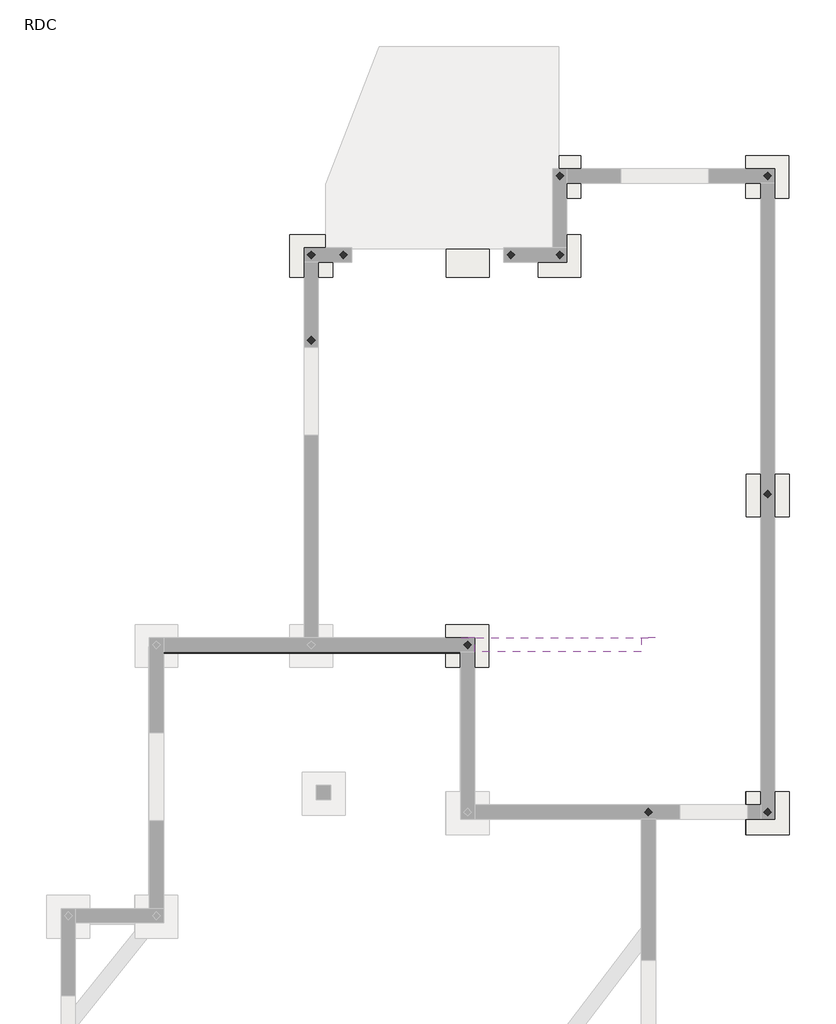
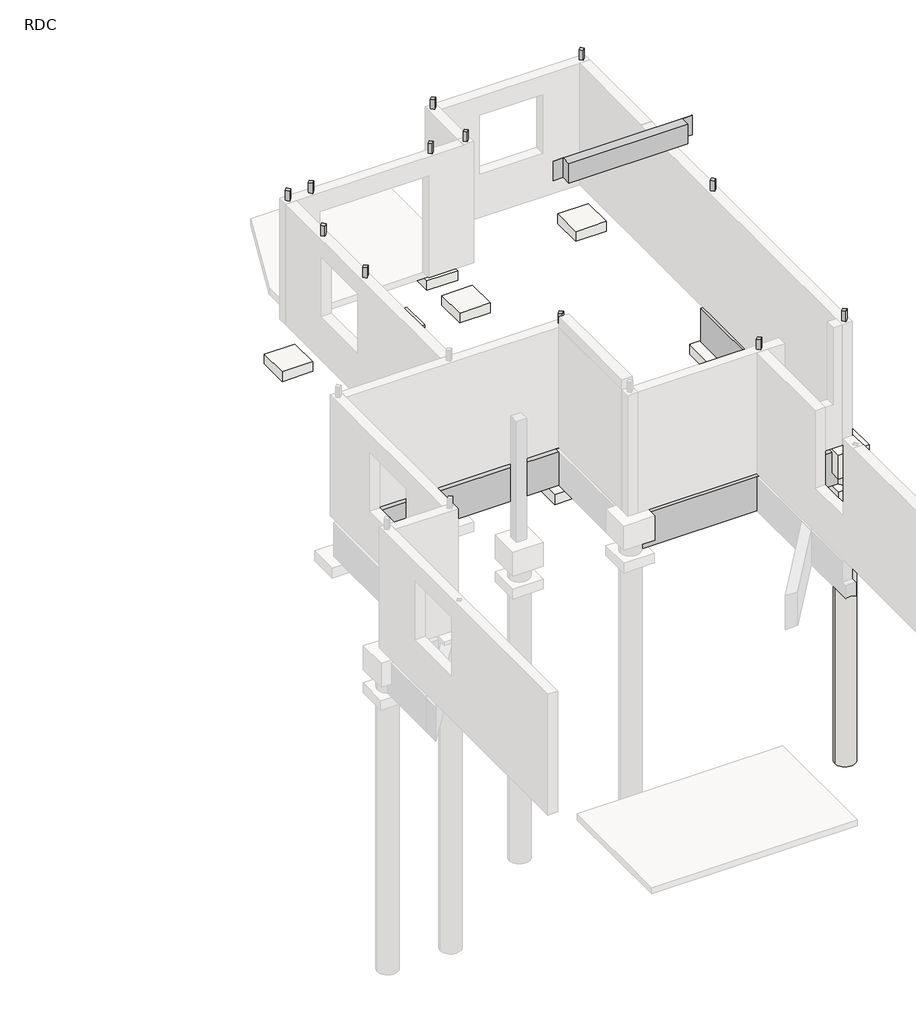
# One storey, part 5 of 5: 12 columns, 10 slabs, 4 beams.
"""IFC4 building model written with IfcOpenShell, lengths in millimetres."""

from ifc_helpers import new_model, si_unit, frame, origin, place, context, project, spatial, polyline, circle_curve, outline, extrude, faceted_brep, element, save
from ifc_brep_helpers import plane_surface, cylinder_surface, revolved_surface, advanced_brep

model = new_model("IFC4")

# Units and contexts
model_context = context("Model", 3, world=origin())
ifc_project = project(units=[si_unit("LENGTHUNIT", "METRE", prefix="MILLI")], contexts=[model_context])

# Site, building, storey
site = spatial("IfcSite", under=ifc_project)
building = spatial("IfcBuilding", under=site)
storey = spatial("IfcBuildingStorey", under=building, Name="RDC", Elevation=0.0)

# Beams
placement = place(None, origin())
element("IfcBeam", 1, ObjectType="Longrine BA : 20x70ht", at=placement, inside=storey, context=model_context, shape_type="AdvancedBrep", body=[
    advanced_brep(
    [(3744.5663998, 5403.8353673, -67.0), (3744.5663998, 5403.8353673, -767.0), (3740.0228667, 5403.8353673, -767.0), (3740.0228667, 5403.8353673, -67.0), (3744.5663998, 808.0224787, -67.0), (3744.5663998, 808.0224787, -500.0), (3744.5663998, 681.2275595, -500.0), (3744.5663998, 681.2275595, -767.0), (3544.5663998, 681.2275595, -767.0), (3544.5663998, 5213.5020686, -767.0), (3740.0228667, 5213.5020686, -767.0), (3544.5663998, 681.2275595, -500.0), (3544.5663998, 808.0224787, -500.0), (3544.5663998, 808.0224787, -67.0), (3544.5663998, 5213.5020686, -67.0), (3740.0228667, 5213.5020686, -67.0)],
    [
        (0, 1),
        (1, 2),
        (2, 3),
        (3, 0),
        (0, 4),
        (4, 5),
        (5, 6),
        (6, 7),
        (7, 1),
        (7, 8, circle_curve(frame((3644.5663998, 508.0224787, -767.0), z_axis=(0.0, 0.0, 1.0), x_axis=(1.0, 0.0, 0.0)), 200.0)),
        (8, 9),
        (9, 10),
        (10, 2),
        (8, 11),
        (11, 12),
        (12, 13),
        (13, 14),
        (14, 9),
        (3, 15),
        (15, 14),
        (13, 4),
        (6, 11, circle_curve(frame((3644.5663998, 508.0224787, -500.0), z_axis=(0.0, 0.0, 1.0), x_axis=(1.0, 0.0, 0.0)), 200.0)),
        (5, 12),
        (10, 15),
    ],
    [
        plane_surface(frame((3744.5663998, 5403.8353673, -67.0), z_axis=(0.0, 1.0, 0.0), x_axis=(0.0, 0.0, -1.0))),
        plane_surface(frame((3744.5663998, 5403.8353673, -417.0), z_axis=(1.0, 0.0, 0.0), x_axis=(0.0, 0.0, -1.0))),
        plane_surface(frame((3644.5663998, 5403.8353673, -767.0), z_axis=(0.0, 0.0, -1.0), x_axis=(-1.0, 0.0, 0.0))),
        plane_surface(frame((3544.5663998, 5403.8353673, -417.0), z_axis=(-1.0, 0.0, 0.0), x_axis=(0.0, 0.0, 1.0))),
        plane_surface(frame((3644.5663998, 5403.8353673, -67.0), z_axis=(0.0, 0.0, 1.0), x_axis=(1.0, 0.0, 0.0))),
        revolved_surface(polyline([(3844.5663998, 508.0224787, -500.0), (3844.5663998, 508.0224787, -767.0)]), (3644.5663998, 508.0224787, -6600.0), (0.0, 0.0, 1.0)),
        plane_surface(frame((3344.5663998, 808.0224787, -500.0), z_axis=(0.0, 0.0, 1.0), x_axis=(1.0, 0.0, 0.0))),
        plane_surface(frame((3944.5663998, 808.0224787, 0.0), z_axis=(0.0, -1.0, 0.0), x_axis=(0.0, 0.0, -1.0))),
        plane_surface(frame((3740.0228667, 9413.5020686, -770.0), z_axis=(-1.0, 0.0, 0.0), x_axis=(0.0, 1.0, 0.0))),
        plane_surface(frame((3540.0228667, 5213.5020686, -770.0), z_axis=(0.0, 1.0, 0.0), x_axis=(1.0, 0.0, 0.0))),
    ],
    [
        (0, [[1, 2, 3, 4]]),
        (1, [[-1, 5, 6, 7, 8, 9]]),
        (2, [[-9, 10, 11, 12, 13, -2]]),
        (3, [[14, 15, 16, 17, 18, -11]]),
        (4, [[-5, -4, 19, 20, -17, 21]]),
        (5, [[-10, -8, 22, -14]]),
        (6, [[23, -15, -22, -7]]),
        (7, [[-23, -6, -21, -16]]),
        (8, [[24, -19, -3, -13]]),
        (9, [[-24, -12, -18, -20]]),
    ],
),
])
element("IfcBeam", 2, ObjectType="Longrine BA : 20x70ht", at=placement, inside=storey, context=model_context, shape_type="AdvancedBrep", body=[
    advanced_brep(
    [(3463.1482907, 423.8353673, -767.0), (3463.1482907, 423.8353673, -500.0), (3344.5663998, 423.8353673, -500.0), (3344.5663998, 423.8353673, -67.0), (2074.5663639, 423.8353673, -67.0), (1874.5663639, 423.8353673, -67.0), (-255.4335965, 423.8353673, -67.0), (-255.4335965, 423.8353673, -500.0), (-374.0154875, 423.8353673, -500.0), (-374.0154875, 423.8353673, -767.0), (1874.5663639, 423.8353673, -767.0), (2074.5663639, 423.8353673, -767.0), (-355.4335965, 508.0224787, -767.0), (-392.3772418, 623.8353673, -767.0), (3481.510045, 623.8353673, -767.0), (3444.5663998, 508.0224787, -767.0), (3481.510045, 623.8353673, -500.0), (-392.3772418, 623.8353673, -500.0), (-255.4335965, 623.8353673, -500.0), (-255.4335965, 623.8353673, -67.0), (3344.5663998, 623.8353673, -67.0), (3344.5663998, 623.8353673, -500.0), (-355.4335965, 508.0224787, -500.0), (3444.5663998, 508.0224787, -500.0)],
    [
        (0, 1),
        (1, 2),
        (2, 3),
        (3, 4),
        (4, 5),
        (5, 6),
        (6, 7),
        (7, 8),
        (8, 9),
        (9, 10),
        (10, 11),
        (11, 0),
        (9, 12, circle_curve(frame((-555.4335965, 508.0224787, -767.0), z_axis=(0.0, 0.0, 1.0), x_axis=(1.0, 0.0, 0.0)), 200.0)),
        (12, 13, circle_curve(frame((-555.4335965, 508.0224787, -767.0), z_axis=(0.0, 0.0, 1.0), x_axis=(1.0, 0.0, 0.0)), 200.0)),
        (13, 14),
        (14, 15, circle_curve(frame((3644.5663998, 508.0224787, -767.0), z_axis=(0.0, 0.0, 1.0), x_axis=(1.0, 0.0, 0.0)), 200.0)),
        (15, 0, circle_curve(frame((3644.5663998, 508.0224787, -767.0), z_axis=(0.0, 0.0, 1.0), x_axis=(1.0, 0.0, 0.0)), 200.0)),
        (16, 14),
        (13, 17),
        (17, 18),
        (18, 19),
        (19, 20),
        (20, 21),
        (21, 16),
        (3, 20),
        (19, 6),
        (8, 22, circle_curve(frame((-555.4335965, 508.0224787, -500.0), z_axis=(0.0, 0.0, 1.0), x_axis=(1.0, 0.0, 0.0)), 200.0)),
        (22, 12),
        (22, 17, circle_curve(frame((-555.4335965, 508.0224787, -500.0), z_axis=(0.0, 0.0, 1.0), x_axis=(1.0, 0.0, 0.0)), 200.0)),
        (15, 23),
        (23, 1, circle_curve(frame((3644.5663998, 508.0224787, -500.0), z_axis=(0.0, 0.0, 1.0), x_axis=(1.0, 0.0, 0.0)), 200.0)),
        (16, 23, circle_curve(frame((3644.5663998, 508.0224787, -500.0), z_axis=(0.0, 0.0, 1.0), x_axis=(1.0, 0.0, 0.0)), 200.0)),
        (21, 2),
        (7, 18),
    ],
    [
        plane_surface(frame((3631.8663992, 423.8353673, -417.0), z_axis=(0.0, -1.0, 0.0), x_axis=(0.0, 0.0, -1.0))),
        plane_surface(frame((3631.8663992, 523.8353673, -767.0), z_axis=(0.0, 0.0, -1.0), x_axis=(0.0, 1.0, 0.0))),
        plane_surface(frame((3631.8663992, 623.8353673, -417.0), z_axis=(0.0, 1.0, 0.0), x_axis=(0.0, 0.0, 1.0))),
        plane_surface(frame((3631.8663992, 523.8353673, -67.0), z_axis=(0.0, 0.0, 1.0), x_axis=(0.0, -1.0, 0.0))),
        revolved_surface(polyline([(-355.4335965, 508.0224787, -500.0), (-355.4335965, 508.0224787, -767.0)]), (-555.4335965, 508.0224787, -6600.0), (0.0, 0.0, 1.0)),
        revolved_surface(polyline([(3844.5663998, 508.0224787, -500.0), (3844.5663998, 508.0224787, -767.0)]), (3644.5663998, 508.0224787, -6600.0), (0.0, 0.0, 1.0)),
        plane_surface(frame((3344.5663998, 808.0224787, -500.0), z_axis=(0.0, 0.0, 1.0), x_axis=(1.0, 0.0, 0.0))),
        plane_surface(frame((3344.5663998, 808.0224787, 0.0), z_axis=(1.0, 0.0, 0.0), x_axis=(0.0, 0.0, -1.0))),
        plane_surface(frame((-855.4335965, 808.0224787, -500.0), z_axis=(0.0, 0.0, 1.0), x_axis=(1.0, 0.0, 0.0))),
        plane_surface(frame((-255.4335965, 208.0224787, 0.0), z_axis=(-1.0, 0.0, 0.0), x_axis=(0.0, 0.0, -1.0))),
    ],
    [
        (0, [[1, 2, 3, 4, 5, 6, 7, 8, 9, 10, 11, 12]]),
        (1, [[13, 14, 15, 16, 17, -12, -11, -10]]),
        (2, [[18, -15, 19, 20, 21, 22, 23, 24]]),
        (3, [[25, -22, 26, -6, -5, -4]]),
        (4, [[-13, -9, 27, 28]]),
        (4, [[-14, -28, 29, -19]]),
        (5, [[-1, -17, 30, 31]]),
        (5, [[-18, 32, -30, -16]]),
        (6, [[33, -2, -31, -32, -24]]),
        (7, [[-33, -23, -25, -3]]),
        (8, [[34, -20, -29, -27, -8]]),
        (9, [[-34, -7, -26, -21]]),
    ],
),
])
element("IfcBeam", 3, ObjectType="Longrine BA : 20x70ht", at=placement, inside=storey, context=model_context, shape_type="Brep", body=[
    faceted_brep([(-4904.4649416, 2948.0224782, -67.0), (-4904.4649416, 2948.0224782, -767.0), (-4904.4649416, 2835.3224776, -767.0), (-4904.4649416, 2835.3224776, -67.0), (-572.6771131, 2948.0224782, -67.0), (-572.6771131, 2835.3224776, -67.0), (-572.6771131, 2748.0224782, -67.0), (-572.6771131, 2748.0224782, -767.0), (-572.6771131, 2835.3224776, -767.0), (-572.6771131, 2948.0224782, -767.0), (-2849.9542111, 2948.0224782, -67.0), (-2849.9542111, 2948.0224782, -767.0), (-659.9771125, 2748.0224782, -767.0), (-4817.1649422, 2748.0224782, -767.0), (-4817.1649422, 2835.3224776, -767.0), (-2849.9542111, 2947.3616236, -767.0), (-2649.9542111, 2947.3616236, -767.0), (-2649.9542111, 2948.0224782, -767.0), (-659.9771125, 2748.0224782, -67.0), (-4817.1649422, 2748.0224782, -67.0), (-2649.9542111, 2948.0224782, -67.0), (-2649.9542111, 2947.3616236, -67.0), (-2849.9542111, 2947.3616236, -67.0), (-4817.1649422, 2835.3224776, -67.0)], [[[0, 1, 2, 3]], [[4, 5, 6, 7, 8, 9]], [[1, 0, 10, 11]], [[9, 8, 7, 12, 13, 14, 2, 1, 11, 15, 16, 17]], [[7, 6, 18, 19, 13, 12]], [[6, 5, 4, 20, 21, 22, 10, 0, 3, 23, 19, 18]], [[23, 14, 13, 19]], [[14, 23, 3, 2]], [[22, 15, 11, 10]], [[15, 22, 21, 16]], [[4, 9, 17, 20]], [[16, 21, 20, 17]]]),
])
element("IfcBeam", 4, ObjectType="Poutres BA : 20x40h", at=placement, inside=storey, context=model_context, shape_type="SweptSolid", body=[
    extrude(outline(polyline([(-645.8307775, 2964.0588408), (2074.1692225, 2964.0588408), (2074.1692225, 2963.8353669), (1874.5663639, 2963.8353669), (1874.5663639, 2764.0588408), (-455.4335965, 2764.0588408), (-455.4335965, 2963.8353669), (-645.8307775, 2963.8353669), (-645.8307775, 2964.0588408)])), frame((0.0, 0.0, 5410.0), z_axis=(0.0, 0.0, 1.0), x_axis=(1.0, 0.0, 0.0)), (0.0, 0.0, 1.0), 400.0),
])

# Columns
element("IfcColumn", 5, ObjectType="CV : CV", at=placement, inside=storey, context=model_context, shape_type="Brep", body=[
    faceted_brep([(-555.4335965, 2916.8683755, 2710.0), (-608.4666051, 2863.8353669, 2710.0), (-555.4335965, 2810.8023583, 2710.0), (-502.4005879, 2863.8353669, 2710.0), (-555.4335965, 2916.8683755, 0.0), (-502.4005879, 2863.8353669, 0.0), (-555.4335965, 2810.8023583, 0.0), (-608.4666051, 2863.8353669, 0.0), (-555.4335965, 2916.8683755, 2500.0), (-608.4666051, 2863.8353669, 2500.0), (-555.4335965, 2810.8023583, 2500.0), (-502.4005879, 2863.8353669, 2500.0)], [[[0, 1, 2, 3]], [[4, 5, 6, 7]], [[1, 0, 8, 4, 7, 9]], [[2, 1, 9, 7, 6, 10]], [[3, 2, 10, 6, 5, 11]], [[0, 3, 11, 5, 4, 8]]]),
    faceted_brep([(-502.4005879, 2863.8353669, 2710.0), (-555.4335965, 2916.8683755, 2710.0), (-608.4666051, 2863.8353669, 2710.0), (-555.4335965, 2810.8023583, 2710.0), (-502.4005879, 2863.8353669, 0.0), (-555.4335965, 2810.8023583, 0.0), (-608.4666051, 2863.8353669, 0.0), (-555.4335965, 2916.8683755, 0.0), (-502.4005879, 2863.8353669, 2500.0), (-555.4335965, 2916.8683755, 2500.0), (-608.4666051, 2863.8353669, 2500.0), (-555.4335965, 2810.8023583, 2500.0)], [[[0, 1, 2, 3]], [[4, 5, 6, 7]], [[1, 0, 8, 4, 7, 9]], [[2, 1, 9, 7, 6, 10]], [[3, 2, 10, 6, 5, 11]], [[0, 3, 11, 5, 4, 8]]]),
])
element("IfcColumn", 6, ObjectType="CV : CV", at=placement, inside=storey, context=model_context, shape_type="Brep", body=[
    faceted_brep([(-2745.4336004, 5751.8684051, 2710.0), (-2798.466609, 5698.8353965, 2710.0), (-2745.4336004, 5645.8023879, 2710.0), (-2692.4005918, 5698.8353965, 2710.0), (-2745.4336004, 5751.8684051, 0.0), (-2692.4005918, 5698.8353965, 0.0), (-2745.4336004, 5645.8023879, 0.0), (-2798.466609, 5698.8353965, 0.0), (-2745.4336004, 5751.8684051, 2500.0), (-2798.466609, 5698.8353965, 2500.0), (-2745.4336004, 5645.8023879, 2500.0), (-2692.4005918, 5698.8353965, 2500.0)], [[[0, 1, 2, 3]], [[4, 5, 6, 7]], [[1, 0, 8, 4, 7, 9]], [[2, 1, 9, 7, 6, 10]], [[3, 2, 10, 6, 5, 11]], [[0, 3, 11, 5, 4, 8]]]),
    faceted_brep([(-2692.4005918, 5698.8353965, 2710.0), (-2745.4336004, 5751.8684051, 2710.0), (-2798.466609, 5698.8353965, 2710.0), (-2745.4336004, 5645.8023879, 2710.0), (-2692.4005918, 5698.8353965, 0.0), (-2745.4336004, 5645.8023879, 0.0), (-2798.466609, 5698.8353965, 0.0), (-2745.4336004, 5751.8684051, 0.0), (-2692.4005918, 5698.8353965, 2500.0), (-2745.4336004, 5751.8684051, 2500.0), (-2798.466609, 5698.8353965, 2500.0), (-2745.4336004, 5645.8023879, 2500.0)], [[[0, 1, 2, 3]], [[4, 5, 6, 7]], [[1, 0, 8, 4, 7, 9]], [[2, 1, 9, 7, 6, 10]], [[3, 2, 10, 6, 5, 11]], [[0, 3, 11, 5, 4, 8]]]),
])
element("IfcColumn", 7, ObjectType="CV : CV", at=placement, inside=storey, context=model_context, shape_type="Brep", body=[
    faceted_brep([(-2745.4336004, 8376.8684051, 2710.0), (-2798.466609, 8323.8353965, 2710.0), (-2745.4336004, 8270.8023879, 2710.0), (-2692.4005918, 8323.8353965, 2710.0), (-2745.4336004, 8376.8684051, 0.0), (-2692.4005918, 8323.8353965, 0.0), (-2745.4336004, 8270.8023879, 0.0), (-2798.466609, 8323.8353965, 0.0), (-2745.4336004, 8376.8684051, 2500.0), (-2798.466609, 8323.8353965, 2500.0), (-2745.4336004, 8270.8023879, 2500.0), (-2692.4005918, 8323.8353965, 2500.0)], [[[0, 1, 2, 3]], [[4, 5, 6, 7]], [[1, 0, 8, 4, 7, 9]], [[2, 1, 9, 7, 6, 10]], [[3, 2, 10, 6, 5, 11]], [[0, 3, 11, 5, 4, 8]]]),
    faceted_brep([(-2692.4005918, 8323.8353965, 2710.0), (-2745.4336004, 8376.8684051, 2710.0), (-2798.466609, 8323.8353965, 2710.0), (-2745.4336004, 8270.8023879, 2710.0), (-2692.4005918, 8323.8353965, 0.0), (-2745.4336004, 8270.8023879, 0.0), (-2798.466609, 8323.8353965, 0.0), (-2745.4336004, 8376.8684051, 0.0), (-2692.4005918, 8323.8353965, 2500.0), (-2745.4336004, 8376.8684051, 2500.0), (-2798.466609, 8323.8353965, 2500.0), (-2745.4336004, 8270.8023879, 2500.0)], [[[0, 1, 2, 3]], [[4, 5, 6, 7]], [[1, 0, 8, 4, 7, 9]], [[2, 1, 9, 7, 6, 10]], [[3, 2, 10, 6, 5, 11]], [[0, 3, 11, 5, 4, 8]]]),
])
element("IfcColumn", 8, ObjectType="CV : CV", at=placement, inside=storey, context=model_context, shape_type="Brep", body=[
    faceted_brep([(-2295.4336038, 8376.8684051, 2710.0), (-2348.4666124, 8323.8353965, 2710.0), (-2295.4336038, 8270.8023879, 2710.0), (-2242.4005953, 8323.8353965, 2710.0), (-2295.4336038, 8376.8684051, 0.0), (-2242.4005953, 8323.8353965, 0.0), (-2295.4336038, 8270.8023879, 0.0), (-2348.4666124, 8323.8353965, 0.0), (-2295.4336038, 8376.8684051, 2500.0), (-2348.4666124, 8323.8353965, 2500.0), (-2295.4336038, 8270.8023879, 2500.0), (-2242.4005953, 8323.8353965, 2500.0)], [[[0, 1, 2, 3]], [[4, 5, 6, 7]], [[1, 0, 8, 4, 7, 9]], [[2, 1, 9, 7, 6, 10]], [[3, 2, 10, 6, 5, 11]], [[0, 3, 11, 5, 4, 8]]]),
    faceted_brep([(-2242.4005953, 8323.8353965, 2710.0), (-2295.4336038, 8376.8684051, 2710.0), (-2348.4666124, 8323.8353965, 2710.0), (-2295.4336038, 8270.8023879, 2710.0), (-2242.4005953, 8323.8353965, 0.0), (-2295.4336038, 8270.8023879, 0.0), (-2348.4666124, 8323.8353965, 0.0), (-2295.4336038, 8376.8684051, 0.0), (-2242.4005953, 8323.8353965, 2500.0), (-2295.4336038, 8376.8684051, 2500.0), (-2348.4666124, 8323.8353965, 2500.0), (-2295.4336038, 8270.8023879, 2500.0)], [[[0, 1, 2, 3]], [[4, 5, 6, 7]], [[1, 0, 8, 4, 7, 9]], [[2, 1, 9, 7, 6, 10]], [[3, 2, 10, 6, 5, 11]], [[0, 3, 11, 5, 4, 8]]]),
])
element("IfcColumn", 9, ObjectType="CV : CV", at=placement, inside=storey, context=model_context, shape_type="Brep", body=[
    faceted_brep([(49.5663962, 8376.8684051, 2710.0), (-3.4666124, 8323.8353965, 2710.0), (49.5663962, 8270.8023879, 2710.0), (102.5994047, 8323.8353965, 2710.0), (49.5663962, 8376.8684051, 0.0), (102.5994047, 8323.8353965, 0.0), (49.5663962, 8270.8023879, 0.0), (-3.4666124, 8323.8353965, 0.0), (49.5663962, 8376.8684051, 2500.0), (-3.4666124, 8323.8353965, 2500.0), (49.5663962, 8270.8023879, 2500.0), (102.5994047, 8323.8353965, 2500.0)], [[[0, 1, 2, 3]], [[4, 5, 6, 7]], [[1, 0, 8, 4, 7, 9]], [[2, 1, 9, 7, 6, 10]], [[3, 2, 10, 6, 5, 11]], [[0, 3, 11, 5, 4, 8]]]),
    faceted_brep([(102.5994047, 8323.8353965, 2710.0), (49.5663962, 8376.8684051, 2710.0), (-3.4666124, 8323.8353965, 2710.0), (49.5663962, 8270.8023879, 2710.0), (102.5994047, 8323.8353965, 0.0), (49.5663962, 8270.8023879, 0.0), (-3.4666124, 8323.8353965, 0.0), (49.5663962, 8376.8684051, 0.0), (102.5994047, 8323.8353965, 2500.0), (49.5663962, 8376.8684051, 2500.0), (-3.4666124, 8323.8353965, 2500.0), (49.5663962, 8270.8023879, 2500.0)], [[[0, 1, 2, 3]], [[4, 5, 6, 7]], [[1, 0, 8, 4, 7, 9]], [[2, 1, 9, 7, 6, 10]], [[3, 2, 10, 6, 5, 11]], [[0, 3, 11, 5, 4, 8]]]),
])
element("IfcColumn", 10, ObjectType="CV : CV", at=placement, inside=storey, context=model_context, shape_type="Brep", body=[
    faceted_brep([(734.5663791, 8376.8684051, 2710.0), (681.5333706, 8323.8353965, 2710.0), (734.5663791, 8270.8023879, 2710.0), (787.5993877, 8323.8353965, 2710.0), (734.5663791, 8376.8684051, 0.0), (787.5993877, 8323.8353965, 0.0), (734.5663791, 8270.8023879, 0.0), (681.5333706, 8323.8353965, 0.0), (734.5663791, 8376.8684051, 2510.0), (681.5333706, 8323.8353965, 2510.0), (734.5663791, 8270.8023879, 2510.0), (787.5993877, 8323.8353965, 2510.0)], [[[0, 1, 2, 3]], [[4, 5, 6, 7]], [[1, 0, 8, 4, 7, 9]], [[2, 1, 9, 7, 6, 10]], [[3, 2, 10, 6, 5, 11]], [[0, 3, 11, 5, 4, 8]]]),
    faceted_brep([(787.5993877, 8323.8353965, 2710.0), (734.5663791, 8376.8684051, 2710.0), (681.5333706, 8323.8353965, 2710.0), (734.5663791, 8270.8023879, 2710.0), (787.5993877, 8323.8353965, 0.0), (734.5663791, 8270.8023879, 0.0), (681.5333706, 8323.8353965, 0.0), (734.5663791, 8376.8684051, 0.0), (787.5993877, 8323.8353965, 2510.0), (734.5663791, 8376.8684051, 2510.0), (681.5333706, 8323.8353965, 2510.0), (734.5663791, 8270.8023879, 2510.0)], [[[0, 1, 2, 3]], [[4, 5, 6, 7]], [[1, 0, 8, 4, 7, 9]], [[2, 1, 9, 7, 6, 10]], [[3, 2, 10, 6, 5, 11]], [[0, 3, 11, 5, 4, 8]]]),
])
element("IfcColumn", 11, ObjectType="CV : CV", at=placement, inside=storey, context=model_context, shape_type="Brep", body=[
    faceted_brep([(734.5663791, 9482.347973, 2710.0), (681.5333706, 9429.3149644, 2710.0), (734.5663791, 9376.2819558, 2710.0), (787.5993877, 9429.3149644, 2710.0), (734.5663791, 9482.347973, 0.0), (787.5993877, 9429.3149644, 0.0), (734.5663791, 9376.2819558, 0.0), (681.5333706, 9429.3149644, 0.0), (734.5663791, 9482.347973, 2510.0), (681.5333706, 9429.3149644, 2510.0), (734.5663791, 9376.2819558, 2510.0), (787.5993877, 9429.3149644, 2510.0)], [[[0, 1, 2, 3]], [[4, 5, 6, 7]], [[1, 0, 8, 4, 7, 9]], [[2, 1, 9, 7, 6, 10]], [[3, 2, 10, 6, 5, 11]], [[0, 3, 11, 5, 4, 8]]]),
    faceted_brep([(787.5993877, 9429.3149644, 2710.0), (734.5663791, 9482.347973, 2710.0), (681.5333706, 9429.3149644, 2710.0), (734.5663791, 9376.2819558, 2710.0), (787.5993877, 9429.3149644, 0.0), (734.5663791, 9376.2819558, 0.0), (681.5333706, 9429.3149644, 0.0), (734.5663791, 9482.347973, 0.0), (787.5993877, 9429.3149644, 2510.0), (734.5663791, 9482.347973, 2510.0), (681.5333706, 9429.3149644, 2510.0), (734.5663791, 9376.2819558, 2510.0)], [[[0, 1, 2, 3]], [[4, 5, 6, 7]], [[1, 0, 8, 4, 7, 9]], [[2, 1, 9, 7, 6, 10]], [[3, 2, 10, 6, 5, 11]], [[0, 3, 11, 5, 4, 8]]]),
])
element("IfcColumn", 12, ObjectType="CV : CV", at=placement, inside=storey, context=model_context, shape_type="Brep", body=[
    faceted_brep([(3644.5663998, 9482.347973, 2710.0), (3591.5333912, 9429.3149644, 2710.0), (3644.5663998, 9376.2819558, 2710.0), (3697.5994084, 9429.3149644, 2710.0), (3644.5663998, 9482.347973, 0.0), (3697.5994084, 9429.3149644, 0.0), (3644.5663998, 9376.2819558, 0.0), (3591.5333912, 9429.3149644, 0.0), (3644.5663998, 9482.347973, 2510.0), (3591.5333912, 9429.3149644, 2510.0), (3644.5663998, 9376.2819558, 2510.0), (3697.5994084, 9429.3149644, 2510.0)], [[[0, 1, 2, 3]], [[4, 5, 6, 7]], [[1, 0, 8, 4, 7, 9]], [[2, 1, 9, 7, 6, 10]], [[3, 2, 10, 6, 5, 11]], [[0, 3, 11, 5, 4, 8]]]),
    faceted_brep([(3697.5994084, 9429.3149644, 2710.0), (3644.5663998, 9482.347973, 2710.0), (3591.5333912, 9429.3149644, 2710.0), (3644.5663998, 9376.2819558, 2710.0), (3697.5994084, 9429.3149644, 0.0), (3644.5663998, 9376.2819558, 0.0), (3591.5333912, 9429.3149644, 0.0), (3644.5663998, 9482.347973, 0.0), (3697.5994084, 9429.3149644, 2510.0), (3644.5663998, 9482.347973, 2510.0), (3591.5333912, 9429.3149644, 2510.0), (3644.5663998, 9376.2819558, 2510.0)], [[[0, 1, 2, 3]], [[4, 5, 6, 7]], [[1, 0, 8, 4, 7, 9]], [[2, 1, 9, 7, 6, 10]], [[3, 2, 10, 6, 5, 11]], [[0, 3, 11, 5, 4, 8]]]),
])
element("IfcColumn", 13, ObjectType="CV : CV", at=placement, inside=storey, context=model_context, shape_type="Brep", body=[
    faceted_brep([(3644.5663998, 5027.347973, 2710.0), (3591.5333912, 4974.3149644, 2710.0), (3644.5663998, 4921.2819558, 2710.0), (3697.5994084, 4974.3149644, 2710.0), (3644.5663998, 5027.347973, 0.0), (3697.5994084, 4974.3149644, 0.0), (3644.5663998, 4921.2819558, 0.0), (3591.5333912, 4974.3149644, 0.0), (3644.5663998, 5027.347973, 2500.0), (3591.5333912, 4974.3149644, 2500.0), (3644.5663998, 4921.2819558, 2500.0), (3697.5994084, 4974.3149644, 2500.0)], [[[0, 1, 2, 3]], [[4, 5, 6, 7]], [[1, 0, 8, 4, 7, 9]], [[2, 1, 9, 7, 6, 10]], [[3, 2, 10, 6, 5, 11]], [[0, 3, 11, 5, 4, 8]]]),
    faceted_brep([(3697.5994084, 4974.3149644, 2710.0), (3644.5663998, 5027.347973, 2710.0), (3591.5333912, 4974.3149644, 2710.0), (3644.5663998, 4921.2819558, 2710.0), (3697.5994084, 4974.3149644, 0.0), (3644.5663998, 4921.2819558, 0.0), (3591.5333912, 4974.3149644, 0.0), (3644.5663998, 5027.347973, 0.0), (3697.5994084, 4974.3149644, 2500.0), (3644.5663998, 5027.347973, 2500.0), (3591.5333912, 4974.3149644, 2500.0), (3644.5663998, 4921.2819558, 2500.0)], [[[0, 1, 2, 3]], [[4, 5, 6, 7]], [[1, 0, 8, 4, 7, 9]], [[2, 1, 9, 7, 6, 10]], [[3, 2, 10, 6, 5, 11]], [[0, 3, 11, 5, 4, 8]]]),
])
element("IfcColumn", 14, ObjectType="CV : CV", at=placement, inside=storey, context=model_context, shape_type="Brep", body=[
    faceted_brep([(3644.5663998, 576.8683759, 2710.0), (3591.5333912, 523.8353673, 2710.0), (3644.5663998, 470.8023588, 2710.0), (3697.5994084, 523.8353673, 2710.0), (3644.5663998, 576.8683759, 0.0), (3697.5994084, 523.8353673, 0.0), (3644.5663998, 470.8023588, 0.0), (3591.5333912, 523.8353673, 0.0), (3644.5663998, 576.8683759, 2500.0), (3591.5333912, 523.8353673, 2500.0), (3644.5663998, 470.8023588, 2500.0), (3697.5994084, 523.8353673, 2500.0)], [[[0, 1, 2, 3]], [[4, 5, 6, 7]], [[1, 0, 8, 4, 7, 9]], [[2, 1, 9, 7, 6, 10]], [[3, 2, 10, 6, 5, 11]], [[0, 3, 11, 5, 4, 8]]]),
    faceted_brep([(3697.5994084, 523.8353673, 2710.0), (3644.5663998, 576.8683759, 2710.0), (3591.5333912, 523.8353673, 2710.0), (3644.5663998, 470.8023588, 2710.0), (3697.5994084, 523.8353673, 0.0), (3644.5663998, 470.8023588, 0.0), (3591.5333912, 523.8353673, 0.0), (3644.5663998, 576.8683759, 0.0), (3697.5994084, 523.8353673, 2500.0), (3644.5663998, 576.8683759, 2500.0), (3591.5333912, 523.8353673, 2500.0), (3644.5663998, 470.8023588, 2500.0)], [[[0, 1, 2, 3]], [[4, 5, 6, 7]], [[1, 0, 8, 4, 7, 9]], [[2, 1, 9, 7, 6, 10]], [[3, 2, 10, 6, 5, 11]], [[0, 3, 11, 5, 4, 8]]]),
])
element("IfcColumn", 15, ObjectType="CV : CV", at=placement, inside=storey, context=model_context, shape_type="Brep", body=[
    faceted_brep([(1974.5663639, 576.8683759, 2710.0), (1921.5333553, 523.8353673, 2710.0), (1974.5663639, 470.8023588, 2710.0), (2027.5993725, 523.8353673, 2710.0), (1974.5663639, 576.8683759, 0.0), (2027.5993725, 523.8353673, 0.0), (1974.5663639, 470.8023588, 0.0), (1921.5333553, 523.8353673, 0.0), (1974.5663639, 576.8683759, 2500.0), (1921.5333553, 523.8353673, 2500.0), (1974.5663639, 470.8023588, 2500.0), (2027.5993725, 523.8353673, 2500.0)], [[[0, 1, 2, 3]], [[4, 5, 6, 7]], [[1, 0, 8, 4, 7, 9]], [[2, 1, 9, 7, 6, 10]], [[3, 2, 10, 6, 5, 11]], [[0, 3, 11, 5, 4, 8]]]),
    faceted_brep([(2027.5993725, 523.8353673, 2710.0), (1974.5663639, 576.8683759, 2710.0), (1921.5333553, 523.8353673, 2710.0), (1974.5663639, 470.8023588, 2710.0), (2027.5993725, 523.8353673, 0.0), (1974.5663639, 470.8023588, 0.0), (1921.5333553, 523.8353673, 0.0), (1974.5663639, 576.8683759, 0.0), (2027.5993725, 523.8353673, 2500.0), (1974.5663639, 576.8683759, 2500.0), (1921.5333553, 523.8353673, 2500.0), (1974.5663639, 470.8023588, 2500.0)], [[[0, 1, 2, 3]], [[4, 5, 6, 7]], [[1, 0, 8, 4, 7, 9]], [[2, 1, 9, 7, 6, 10]], [[3, 2, 10, 6, 5, 11]], [[0, 3, 11, 5, 4, 8]]]),
])
element("IfcColumn", 16, ObjectType="CV : CV", at=placement, inside=storey, context=model_context, shape_type="Brep", body=[
    faceted_brep([(-2745.4336004, 7181.0121016, 2710.0), (-2798.466609, 7127.979093, 2710.0), (-2745.4336004, 7074.9460844, 2710.0), (-2692.4005918, 7127.979093, 2710.0), (-2745.4336004, 7181.0121016, 0.0), (-2692.4005918, 7127.979093, 0.0), (-2745.4336004, 7074.9460844, 0.0), (-2798.466609, 7127.979093, 0.0), (-2745.4336004, 7181.0121016, 2500.0), (-2798.466609, 7127.979093, 2500.0), (-2745.4336004, 7074.9460844, 2500.0), (-2692.4005918, 7127.979093, 2500.0)], [[[0, 1, 2, 3]], [[4, 5, 6, 7]], [[1, 0, 8, 4, 7, 9]], [[2, 1, 9, 7, 6, 10]], [[3, 2, 10, 6, 5, 11]], [[0, 3, 11, 5, 4, 8]]]),
    faceted_brep([(-2692.4005918, 7127.979093, 2710.0), (-2745.4336004, 7181.0121016, 2710.0), (-2798.466609, 7127.979093, 2710.0), (-2745.4336004, 7074.9460844, 2710.0), (-2692.4005918, 7127.979093, 0.0), (-2745.4336004, 7074.9460844, 0.0), (-2798.466609, 7127.979093, 0.0), (-2745.4336004, 7181.0121016, 0.0), (-2692.4005918, 7127.979093, 2500.0), (-2745.4336004, 7181.0121016, 2500.0), (-2798.466609, 7127.979093, 2500.0), (-2745.4336004, 7074.9460844, 2500.0)], [[[0, 1, 2, 3]], [[4, 5, 6, 7]], [[1, 0, 8, 4, 7, 9]], [[2, 1, 9, 7, 6, 10]], [[3, 2, 10, 6, 5, 11]], [[0, 3, 11, 5, 4, 8]]]),
])

# Slabs
element("IfcSlab", 17, ObjectType="Pieu-Conduite en acier : Diamètre de 400 mm", at=placement, inside=storey, context=model_context, shape_type="AdvancedBrep", body=[
    advanced_brep(
    [(3444.5663998, 508.0224787, -6600.0), (3844.5663998, 508.0224787, -6600.0), (3444.5663998, 508.0224787, -970.0), (3844.5663998, 508.0224787, -970.0)],
    [
        (0, 1, circle_curve(frame((3644.5663998, 508.0224787, -6600.0), z_axis=(0.0, 0.0, -1.0), x_axis=(1.0, 0.0, 0.0)), 200.0)),
        (1, 0, circle_curve(frame((3644.5663998, 508.0224787, -6600.0), z_axis=(0.0, 0.0, -1.0), x_axis=(1.0, 0.0, 0.0)), 200.0)),
        (2, 3, circle_curve(frame((3644.5663998, 508.0224787, -970.0), z_axis=(0.0, 0.0, 1.0), x_axis=(1.0, 0.0, 0.0)), 200.0)),
        (3, 2, circle_curve(frame((3644.5663998, 508.0224787, -970.0), z_axis=(0.0, 0.0, 1.0), x_axis=(1.0, 0.0, 0.0)), 200.0)),
        (1, 3),
        (2, 0),
    ],
    [
        plane_surface(frame((3844.5663998, 508.0224787, -6600.0), z_axis=(0.0, 0.0, -1.0), x_axis=(0.0, -1.0, 0.0))),
        plane_surface(frame((3340.0228502, 808.0224787, -970.0), z_axis=(0.0, 0.0, 1.0), x_axis=(1.0, 0.0, 0.0))),
        cylinder_surface(frame((3644.5663998, 508.0224787, -6600.0), z_axis=(0.0, 0.0, 1.0), x_axis=(1.0, 0.0, 0.0)), 200.0),
    ],
    [
        (0, [[1, 2]]),
        (1, [[3, 4]]),
        (2, [[-2, 5, -3, 6]]),
        (2, [[-1, -6, -4, -5]]),
    ],
),
    advanced_brep(
    [(3444.5663998, 508.0224787, -770.0), (3844.5663998, 508.0224787, -770.0), (3844.5663998, 508.0224787, -500.0), (3463.1482907, 423.8353673, -500.0), (3444.5663998, 508.0224787, -500.0), (3481.5169902, 623.845145, -500.0), (3544.5663998, 681.2275595, -500.0), (3744.5663998, 681.2275595, -500.0)],
    [
        (0, 1, circle_curve(frame((3644.5663998, 508.0224787, -770.0), z_axis=(0.0, 0.0, 1.0), x_axis=(1.0, 0.0, 0.0)), 200.0)),
        (1, 2),
        (2, 3, circle_curve(frame((3644.5663998, 508.0224787, -500.0), z_axis=(0.0, 0.0, -1.0), x_axis=(1.0, 0.0, 0.0)), 200.0)),
        (3, 4, circle_curve(frame((3644.5663998, 508.0224787, -500.0), z_axis=(0.0, 0.0, -1.0), x_axis=(1.0, 0.0, 0.0)), 200.0)),
        (4, 0),
        (1, 0, circle_curve(frame((3644.5663998, 508.0224787, -770.0), z_axis=(0.0, 0.0, 1.0), x_axis=(1.0, 0.0, 0.0)), 200.0)),
        (4, 5, circle_curve(frame((3644.5663998, 508.0224787, -500.0), z_axis=(0.0, 0.0, -1.0), x_axis=(1.0, 0.0, 0.0)), 200.0)),
        (5, 6, circle_curve(frame((3644.5663998, 508.0224787, -500.0), z_axis=(0.0, 0.0, -1.0), x_axis=(1.0, 0.0, 0.0)), 200.0)),
        (6, 7, circle_curve(frame((3644.5663998, 508.0224787, -500.0), z_axis=(0.0, 0.0, -1.0), x_axis=(1.0, 0.0, 0.0)), 200.0)),
        (7, 2, circle_curve(frame((3644.5663998, 508.0224787, -500.0), z_axis=(0.0, 0.0, -1.0), x_axis=(1.0, 0.0, 0.0)), 200.0)),
    ],
    [
        cylinder_surface(frame((3644.5663998, 508.0224787, -6600.0), z_axis=(0.0, 0.0, 1.0), x_axis=(1.0, 0.0, 0.0)), 200.0),
        plane_surface(frame((3340.0228502, 808.0224787, -770.0), z_axis=(0.0, 0.0, -1.0), x_axis=(-1.0, 0.0, 0.0))),
        plane_surface(frame((3344.5663998, 808.0224787, -500.0), z_axis=(0.0, 0.0, 1.0), x_axis=(1.0, 0.0, 0.0))),
    ],
    [
        (0, [[1, 2, 3, 4, 5]]),
        (0, [[6, -5, 7, 8, 9, 10, -2]]),
        (1, [[-1, -6]]),
        (2, [[-4, -3, -10, -9, -8, -7]]),
    ],
),
])
element("IfcSlab", 18, ObjectType="Tête de pieux-1 poteau : 60x60x50", at=placement, inside=storey, context=model_context, shape_type="Brep", body=[
    faceted_brep([(3944.5663998, 808.0224787, 0.0), (3344.5663998, 808.0224787, 0.0), (3344.5663998, 208.0224787, 0.0), (3944.5663998, 208.0224787, 0.0), (3944.5663998, 808.0224787, -500.0), (3944.5663998, 208.0224787, -500.0), (3344.5663998, 208.0224787, -500.0), (3344.5663998, 423.8353673, -500.0), (3344.5663998, 623.8353673, -500.0), (3344.5663998, 808.0224787, -500.0), (3544.5663998, 808.0224787, -500.0), (3744.5663998, 808.0224787, -500.0)], [[[0, 1, 2, 3]], [[4, 5, 6, 7, 8, 9, 10, 11]], [[1, 0, 4, 11, 10, 9]], [[2, 1, 9, 8, 7, 6]], [[3, 2, 6, 5]], [[0, 3, 5, 4]]]),
])
element("IfcSlab", 19, ObjectType="M_Base-Rectangulaire : 60x60x20", at=placement, inside=storey, context=model_context, shape_type="Brep", body=[
    faceted_brep([(-2445.4336004, 8608.0224784, -770.0), (-3045.4336004, 8608.0224784, -770.0), (-3045.4336004, 8008.0224784, -770.0), (-2449.9542111, 8008.0224784, -770.0), (-2445.4336004, 8008.0224784, -770.0), (-2445.4336004, 8608.0224784, -970.0), (-2445.4336004, 8008.0224784, -970.0), (-2449.9542111, 8008.0224784, -970.0), (-3045.4336004, 8008.0224784, -970.0), (-3045.4336004, 8608.0224784, -970.0)], [[[0, 1, 2, 3, 4]], [[5, 6, 7, 8, 9]], [[1, 0, 5, 9]], [[2, 1, 9, 8]], [[4, 3, 2, 8, 7, 6]], [[0, 4, 6, 5]]]),
    faceted_brep([(-2445.4336004, 8608.0224784, -770.0), (-3045.4336004, 8608.0224784, -770.0), (-3045.4336004, 8008.0224784, -770.0), (-2449.9542111, 8008.0224784, -770.0), (-2445.4336004, 8008.0224784, -770.0), (-2445.4336004, 8608.0224784, -970.0), (-2445.4336004, 8008.0224784, -970.0), (-2449.9542111, 8008.0224784, -970.0), (-3045.4336004, 8008.0224784, -970.0), (-3045.4336004, 8608.0224784, -970.0)], [[[0, 1, 2, 3, 4]], [[5, 6, 7, 8, 9]], [[1, 0, 5, 9]], [[2, 1, 9, 8]], [[4, 3, 2, 8, 7, 6]], [[0, 4, 6, 5]]]),
])
element("IfcSlab", 20, ObjectType="M_Base-Rectangulaire : 60x60x20", at=placement, inside=storey, context=model_context, shape_type="SweptSolid", body=[
    extrude(outline(polyline([(-255.4335965, 8608.0224784), (-255.4335965, 8008.0224784), (-855.4335965, 8008.0224784), (-855.4335965, 8608.0224784), (-255.4335965, 8608.0224784)])), frame((0.0, 0.0, -970.0), z_axis=(0.0, 0.0, 1.0), x_axis=(1.0, 0.0, 0.0)), (0.0, 0.0, 1.0), 200.0),
    extrude(outline(polyline([(-255.4335965, 8608.0224784), (-255.4335965, 8008.0224784), (-855.4335965, 8008.0224784), (-855.4335965, 8608.0224784), (-255.4335965, 8608.0224784)])), frame((0.0, 0.0, -970.0), z_axis=(0.0, 0.0, 1.0), x_axis=(1.0, 0.0, 0.0)), (0.0, 0.0, 1.0), 200.0),
])
element("IfcSlab", 21, ObjectType="M_Base-Rectangulaire : 60x60x20", at=placement, inside=storey, context=model_context, shape_type="SweptSolid", body=[
    extrude(outline(polyline([(1030.0228631, 8608.0224784), (1030.0228631, 8008.0224784), (430.0228631, 8008.0224784), (430.0228631, 8608.0224784), (1030.0228631, 8608.0224784)])), frame((0.0, 0.0, -970.0), z_axis=(0.0, 0.0, 1.0), x_axis=(1.0, 0.0, 0.0)), (0.0, 0.0, 1.0), 200.0),
    extrude(outline(polyline([(1030.0228631, 8608.0224784), (1030.0228631, 8008.0224784), (430.0228631, 8008.0224784), (430.0228631, 8608.0224784), (1030.0228631, 8608.0224784)])), frame((0.0, 0.0, -970.0), z_axis=(0.0, 0.0, 1.0), x_axis=(1.0, 0.0, 0.0)), (0.0, 0.0, 1.0), 200.0),
])
element("IfcSlab", 22, ObjectType="M_Base-Rectangulaire : 60x60x20", at=placement, inside=storey, context=model_context, shape_type="SweptSolid", body=[
    extrude(outline(polyline([(1030.0228631, 9713.5020686), (1030.0228631, 9113.5020686), (430.0228631, 9113.5020686), (430.0228631, 9713.5020686), (1030.0228631, 9713.5020686)])), frame((0.0, 0.0, -970.0), z_axis=(0.0, 0.0, 1.0), x_axis=(1.0, 0.0, 0.0)), (0.0, 0.0, 1.0), 200.0),
    extrude(outline(polyline([(1030.0228631, 9713.5020686), (1030.0228631, 9113.5020686), (430.0228631, 9113.5020686), (430.0228631, 9713.5020686), (1030.0228631, 9713.5020686)])), frame((0.0, 0.0, -970.0), z_axis=(0.0, 0.0, 1.0), x_axis=(1.0, 0.0, 0.0)), (0.0, 0.0, 1.0), 200.0),
])
element("IfcSlab", 23, ObjectType="M_Base-Rectangulaire : 60x60x20", at=placement, inside=storey, context=model_context, shape_type="SweptSolid", body=[
    extrude(outline(polyline([(3940.0228667, 9713.5020686), (3940.0228667, 9113.5020686), (3340.0228667, 9113.5020686), (3340.0228667, 9713.5020686), (3940.0228667, 9713.5020686)])), frame((0.0, 0.0, -970.0), z_axis=(0.0, 0.0, 1.0), x_axis=(1.0, 0.0, 0.0)), (0.0, 0.0, 1.0), 200.0),
    extrude(outline(polyline([(3940.0228667, 9713.5020686), (3940.0228667, 9113.5020686), (3340.0228667, 9113.5020686), (3340.0228667, 9713.5020686), (3940.0228667, 9713.5020686)])), frame((0.0, 0.0, -970.0), z_axis=(0.0, 0.0, 1.0), x_axis=(1.0, 0.0, 0.0)), (0.0, 0.0, 1.0), 200.0),
])
element("IfcSlab", 24, ObjectType="M_Base-Rectangulaire : 60x60x20", at=placement, inside=storey, context=model_context, shape_type="Brep", body=[
    faceted_brep([(3944.5663998, 5255.0521049, -770.0), (3940.0228667, 5255.0521049, -770.0), (3344.5663998, 5255.0521049, -770.0), (3344.5663998, 5213.5020686, -770.0), (3344.5663998, 4655.0521049, -770.0), (3944.5663998, 4655.0521049, -770.0), (3944.5663998, 5255.0521049, -970.0), (3944.5663998, 4655.0521049, -970.0), (3344.5663998, 4655.0521049, -970.0), (3344.5663998, 5213.5020686, -970.0), (3344.5663998, 5255.0521049, -970.0), (3940.0228667, 5255.0521049, -970.0)], [[[0, 1, 2, 3, 4, 5]], [[6, 7, 8, 9, 10, 11]], [[2, 1, 0, 6, 11, 10]], [[4, 3, 2, 10, 9, 8]], [[5, 4, 8, 7]], [[0, 5, 7, 6]]]),
    faceted_brep([(3944.5663998, 5255.0521049, -770.0), (3940.0228667, 5255.0521049, -770.0), (3344.5663998, 5255.0521049, -770.0), (3344.5663998, 5213.5020686, -770.0), (3344.5663998, 4655.0521049, -770.0), (3944.5663998, 4655.0521049, -770.0), (3944.5663998, 5255.0521049, -970.0), (3944.5663998, 4655.0521049, -970.0), (3344.5663998, 4655.0521049, -970.0), (3344.5663998, 5213.5020686, -970.0), (3344.5663998, 5255.0521049, -970.0), (3940.0228667, 5255.0521049, -970.0)], [[[0, 1, 2, 3, 4, 5]], [[6, 7, 8, 9, 10, 11]], [[2, 1, 0, 6, 11, 10]], [[4, 3, 2, 10, 9, 8]], [[5, 4, 8, 7]], [[0, 5, 7, 6]]]),
])
element("IfcSlab", 25, ObjectType="M_Base-Rectangulaire : 60x60x20", at=placement, inside=storey, context=model_context, shape_type="SweptSolid", body=[
    extrude(outline(polyline([(3940.0228502, 808.0224787), (3940.0228502, 208.0224787), (3340.0228502, 208.0224787), (3340.0228502, 808.0224787), (3940.0228502, 808.0224787)])), frame((0.0, 0.0, -970.0), z_axis=(0.0, 0.0, 1.0), x_axis=(1.0, 0.0, 0.0)), (0.0, 0.0, 1.0), 200.0),
    extrude(outline(polyline([(3940.0228502, 808.0224787), (3940.0228502, 208.0224787), (3340.0228502, 208.0224787), (3340.0228502, 808.0224787), (3940.0228502, 808.0224787)])), frame((0.0, 0.0, -970.0), z_axis=(0.0, 0.0, 1.0), x_axis=(1.0, 0.0, 0.0)), (0.0, 0.0, 1.0), 200.0),
])
element("IfcSlab", 26, ObjectType="M_Base-Rectangulaire : 60x60x20", at=placement, inside=storey, context=model_context, shape_type="SweptSolid", body=[
    extrude(outline(polyline([(-259.9771125, 3148.0224782), (-259.9771125, 2548.0224782), (-859.9771125, 2548.0224782), (-859.9771125, 3148.0224782), (-259.9771125, 3148.0224782)])), frame((0.0, 0.0, -970.0), z_axis=(0.0, 0.0, 1.0), x_axis=(1.0, 0.0, 0.0)), (0.0, 0.0, 1.0), 200.0),
    extrude(outline(polyline([(-259.9771125, 3148.0224782), (-259.9771125, 2548.0224782), (-859.9771125, 2548.0224782), (-859.9771125, 3148.0224782), (-259.9771125, 3148.0224782)])), frame((0.0, 0.0, -970.0), z_axis=(0.0, 0.0, 1.0), x_axis=(1.0, 0.0, 0.0)), (0.0, 0.0, 1.0), 200.0),
])

save(model, "model.ifc")

# Revit data of these elements
# Type "Longrine BA : 20x70ht"
#   Length [instance default] = 1.524 m
#   b = 0.200 m
#   h = 0.700 m
#   Structural Material = Maçonnerie - Béton
#   Assembly Code = ""
# Type "Poutres BA : 20x40h"
#   Length [instance default] = 1.524 m
#   b = 0.200 m
#   h = 0.400 m
#   Structural Material = Maçonnerie - Béton
#   Assembly Code = ""
# Type "CV : CV"
#   Structural Material [instance default] = Béton coulé sur place
#   Default Elevation = 0
# Type "Pieu-Conduite en acier : Diamètre de 400 mm"
#   Assembly Code = "A1020130"
#   Rayon = 0.200 m
#   Enrobage minimum = 0.150 m
#   Diameter = 0.400 m
#   Depth = 6.000 m
#   Structural Material [instance default] = Métal - Acier - 345 MPa
# Type "Tête de pieux-1 poteau : 60x60x50"
#   Assembly Code = "A1010130"
#   Width = 0.600 m
#   Length = 0.600 m
#   Foundation Thickness = 0.500 m
#   Coupure = 0.050 m
#   Structural Material [instance default] = Béton - Béton coulé sur place
#   Type de pieu = Pieu-Conduite en acier : Diamètre de 400 mm
# Type "M_Base-Rectangulaire : 60x60x20"
#   Length = 0.600 m
#   Width = 0.600 m
#   Foundation Thickness = 0.200 m
#   Structural Material [instance default] = Béton - Béton coulé sur place
#   Assembly Code = ""
# Elements 1, 2, 3 (IfcBeam, "Longrine BA : 20x70ht")
#   Phase Created = Nouvelle construction
#   Materials on its faces: "Maçonnerie - Béton"
# Element 4 (IfcBeam, "Poutres BA : 20x40h")
#   Phase Created = Nouvelle construction
#   Materials on its faces: "Maçonnerie - Béton"
# Elements 5, 6, 7, 8, 9, 10, 11, 12, 13, 14, 15, 16 (IfcColumn, "CV : CV")
#   Structural Material = Béton coulé sur place
#   Phase Created = Nouvelle construction
#   Materials on its faces: "Béton coulé sur place"
# Element 17 (IfcSlab, "Pieu-Conduite en acier : Diamètre de 400 mm")
#   Structural Material = none
#   Phase Created = Nouvelle construction
# Element 18 (IfcSlab, "Tête de pieux-1 poteau : 60x60x50")
#   Structural Material = Béton - Béton coulé sur place
#   Phase Created = Nouvelle construction
#   Materials on its faces: "Béton - Béton coulé sur place"
# Elements 19, 20, 21, 22, 23, 24, 25, 26 (IfcSlab, "M_Base-Rectangulaire : 60x60x20")
#   Structural Material = Béton - Béton coulé sur place
#   Phase Created = Nouvelle construction
#   Materials on its faces: "Béton - Béton coulé sur place"
# Materials
#   "Maçonnerie - Béton": class "Béton", colour RGB 153 162 160, transparency 0, Cost = 0
#   "Béton coulé sur place": class "Béton", colour RGB 0 0 0, transparency 0, Description = "Matériau physique.", Cost = 0
#   "Métal - Acier - 345 MPa": class "Métal", colour RGB 247 247 247, transparency 0, Cost = 0
#   "Béton - Béton coulé sur place": class "Béton", colour RGB 192 192 192, transparency 0, Cost = 0
